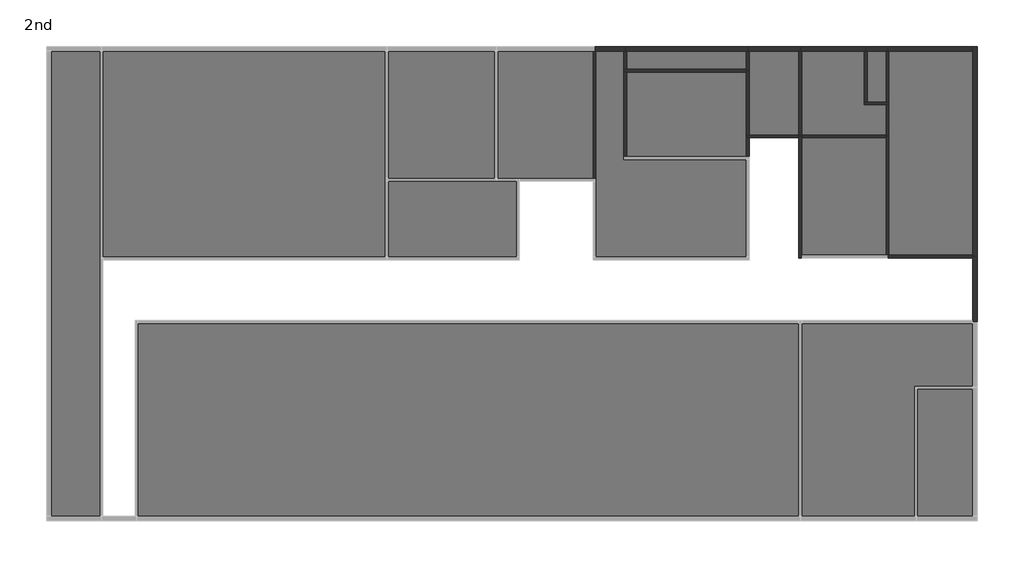
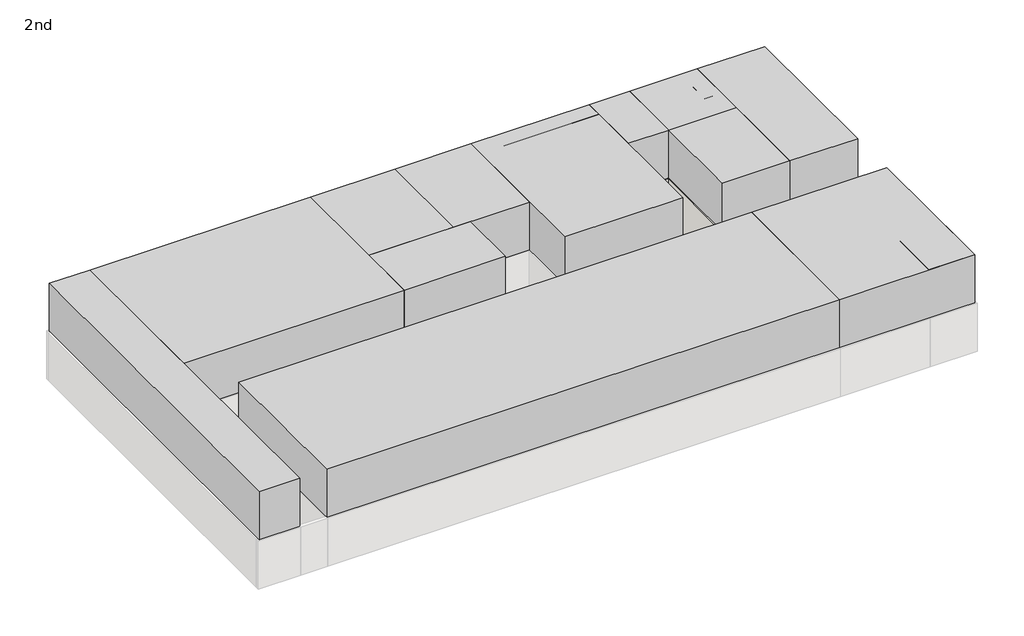
# One storey, part 2 of 2: 42 walls, 17 proxies.
"""IFC4 building model written with IfcOpenShell, lengths in millimetres."""

import ifcopenshell
import ifcopenshell.guid

model = None  # the IFC model being written
_history = None  # IfcOwnerHistory: only IFC2X3 demands one
_inside = {}  # id of a spatial element -> (the spatial element, [elements in it])
_under = {}  # id of a project, library or spatial element -> (it, [spatial elements below it])
_declared = {}  # id of a project -> (the project, [libraries it declares])
_typed = {}  # id of a type object -> (the type object, [elements of that type])
_made_of = {}  # id of a material, layer set ... -> (it, [elements and type objects made of it])


def new_model(schema):
    """Start an empty IFC model of exactly this schema.

    Asked for "IFC4X3", IfcOpenShell would pick the latest addendum, in which some entities
    have other attributes; the version numbers below select the first issue.
    IFC2X3 requires an IfcOwnerHistory on every rooted entity: one is made here for all.
    """
    global model, _history
    if schema == "IFC4X3":
        model = ifcopenshell.file(schema_version=(4, 3, 0, 0))
    else:
        model = ifcopenshell.file(schema=schema)
    _inside.clear()
    _under.clear()
    _declared.clear()
    _typed.clear()
    _made_of.clear()
    _history = None
    if model.schema == "IFC2X3":
        org = make("IfcOrganization", Name="unknown")
        user = make(
            "IfcPersonAndOrganization",
            ThePerson=make("IfcPerson", FamilyName="unknown"),
            TheOrganization=org,
        )
        app = make(
            "IfcApplication",
            ApplicationDeveloper=org,
            Version="unknown",
            ApplicationFullName="unknown",
            ApplicationIdentifier="unknown",
        )
        _history = make(
            "IfcOwnerHistory",
            OwningUser=user,
            OwningApplication=app,
            ChangeAction="ADDED",
            CreationDate=0,
        )
    return model


def make(cls, **values):
    """One entity of the class cls with the attributes given. An attribute that is None is left unset."""
    return model.create_entity(
        cls, **{name: value for name, value in values.items() if value is not None}
    )


def rooted(cls, **values):
    """An entity with a GlobalId (a new one), such as an element, a storey or a relation."""
    return make(cls, GlobalId=ifcopenshell.guid.new(), OwnerHistory=_history, **values)


def si_unit(unit_type, name, prefix=None):
    """IfcSIUnit, for example si_unit("LENGTHUNIT", "METRE", prefix="MILLI")."""
    return make("IfcSIUnit", UnitType=unit_type, Prefix=prefix, Name=name)


def assignment(units):
    """IfcUnitAssignment: the units of a project."""
    return None if units is None else make("IfcUnitAssignment", Units=units)


def point(xyz):
    """IfcCartesianPoint."""
    return None if xyz is None else make("IfcCartesianPoint", Coordinates=xyz)


def direction(xyz):
    """IfcDirection."""
    return None if xyz is None else make("IfcDirection", DirectionRatios=xyz)


def frame(location, z_axis=None, x_axis=None):
    """IfcAxis2Placement3D, a coordinate frame: its origin and axes. An axis left out is left unset."""
    return make(
        "IfcAxis2Placement3D",
        Location=point(location),
        Axis=direction(z_axis),
        RefDirection=direction(x_axis),
    )


def origin():
    """The frame at (0, 0, 0) with its axes left unset."""
    return frame((0.0, 0.0, 0.0))


def origin_with_axes():
    """The frame at (0, 0, 0) with the z axis (0, 0, 1) and the x axis (1, 0, 0) written out."""
    return frame((0.0, 0.0, 0.0), z_axis=(0.0, 0.0, 1.0), x_axis=(1.0, 0.0, 0.0))


def place(relative_to, where):
    """IfcLocalPlacement: puts the frame where relative to a parent placement (None: the world)."""
    return make(
        "IfcLocalPlacement", PlacementRelTo=relative_to, RelativePlacement=where
    )


def context(
    kind, dimensions, precision=None, world=None, true_north=None, identifier=None
):
    """IfcGeometricRepresentationContext, for example the 3D "Model" context."""
    return make(
        "IfcGeometricRepresentationContext",
        ContextIdentifier=identifier,
        ContextType=kind,
        CoordinateSpaceDimension=dimensions,
        Precision=precision,
        WorldCoordinateSystem=world,
        TrueNorth=true_north,
    )


def project(units=None, contexts=None):
    """IfcProject with its units and contexts."""
    return rooted(
        "IfcProject",
        Name="project",
        RepresentationContexts=contexts,
        UnitsInContext=assignment(units),
    )


def spatial(cls, under=None, at=None, **own):
    """A site, building, storey or space (cls), placed at a placement, below another one or the project."""
    s = rooted(cls, ObjectPlacement=at, **own)
    if under is not None:
        _under.setdefault(under.id(), (under, []))[1].append(s)
    return s


def polyline(points):
    """IfcPolyline through the points."""
    return make("IfcPolyline", Points=[point(p) for p in points])


def outline(outer, holes=None, kind="AREA"):
    """IfcArbitraryClosedProfileDef: a profile drawn as a closed curve; with holes, ...WithVoids."""
    if holes is None:
        return make("IfcArbitraryClosedProfileDef", ProfileType=kind, OuterCurve=outer)
    return make(
        "IfcArbitraryProfileDefWithVoids",
        ProfileType=kind,
        OuterCurve=outer,
        InnerCurves=holes,
    )


def extrude(swept, where, along, depth):
    """IfcExtrudedAreaSolid: the profile swept, set in the frame where, extruded along a direction by depth."""
    return make(
        "IfcExtrudedAreaSolid",
        SweptArea=swept,
        Position=where,
        ExtrudedDirection=direction(along),
        Depth=depth,
    )


def faces_of(points, faces, orient=None, outer=None):
    """IfcFace entities. A face is a list of loops; a loop is a list of indices into points, from 0.

    orient and outer hold one flag for each loop. By default every Orientation is true, the
    first loop of a face is its IfcFaceOuterBound and the others are IfcFaceBound.
    """
    made = []
    for i, loops in enumerate(faces):
        bounds = []
        for j, loop in enumerate(loops):
            is_outer = j == 0 if outer is None else outer[i][j]
            bounds.append(
                make(
                    "IfcFaceOuterBound" if is_outer else "IfcFaceBound",
                    Bound=make("IfcPolyLoop", Polygon=[points[k] for k in loop]),
                    Orientation=True if orient is None else orient[i][j],
                )
            )
        made.append(make("IfcFace", Bounds=bounds))
    return made


def faceted_brep(points, faces, orient=None, outer=None, voids=None):
    """IfcFacetedBrep: a solid bounded by flat faces; with voids (closed shells), ...WithVoids."""
    shared = [point(p) for p in points]
    hull = make("IfcClosedShell", CfsFaces=faces_of(shared, faces, orient, outer))
    if voids is None:
        return make("IfcFacetedBrep", Outer=hull)
    return make(
        "IfcFacetedBrepWithVoids",
        Outer=hull,
        Voids=[
            make(cls, CfsFaces=faces_of(shared, fs, o, b)) for cls, fs, o, b in voids
        ],
    )


def shape(context_of_items, identifier, shape_type, items):
    """IfcShapeRepresentation: the items that make up one representation, for example the "Body"."""
    return make(
        "IfcShapeRepresentation",
        ContextOfItems=context_of_items,
        RepresentationIdentifier=identifier,
        RepresentationType=shape_type,
        Items=items,
    )


def source(mapping_origin, context_of_items, identifier, shape_type, items):
    """IfcRepresentationMap: a shape defined once, which mapped items show again and again."""
    return make(
        "IfcRepresentationMap",
        MappingOrigin=mapping_origin,
        MappedRepresentation=shape(context_of_items, identifier, shape_type, items),
    )


def transform(
    local_origin,
    x_axis=None,
    y_axis=None,
    z_axis=None,
    scale=None,
    scale2=None,
    scale3=None,
    uniform=True,
):
    """IfcCartesianTransformationOperator3D, or its non-uniform kind. x_axis, y_axis, z_axis: its Axis1, 2, 3."""
    if uniform:
        return make(
            "IfcCartesianTransformationOperator3D",
            Axis1=direction(x_axis),
            Axis2=direction(y_axis),
            LocalOrigin=point(local_origin),
            Scale=scale,
            Axis3=direction(z_axis),
        )
    return make(
        "IfcCartesianTransformationOperator3DnonUniform",
        Axis1=direction(x_axis),
        Axis2=direction(y_axis),
        LocalOrigin=point(local_origin),
        Scale=scale,
        Axis3=direction(z_axis),
        Scale2=scale2,
        Scale3=scale3,
    )


def mapped(mapping_source, mapping_target):
    """IfcMappedItem: shows the shape of a source again, moved by a transform."""
    return make(
        "IfcMappedItem", MappingSource=mapping_source, MappingTarget=mapping_target
    )


def made_of(thing, what):
    """Note that an element or type object is made of a material, layer set ...; save() writes the relation."""
    if what is not None:
        _made_of.setdefault(what.id(), (what, []))[1].append(thing)
    return thing


def element(
    cls,
    number,
    at=None,
    inside=None,
    cuts=None,
    type_object=None,
    material=None,
    context=None,
    identifier="Body",
    shape_type=None,
    held_by="IfcProductDefinitionShape",
    body=None,
    shapes=None,
    **own,
):
    """One element of the class cls, such as IfcWall. Its Tag is "e" and its number.

    at: its placement. inside: the storey or other place that contains it. cuts: it is an
    opening in that element (IfcRelVoidsElement). A single representation is given by context,
    identifier, shape_type and body (its items); several are given by shapes. held_by: the class
    of the entity that holds the representations. save() writes the other relations.
    """
    e = rooted(cls, Tag="e%d" % number, ObjectPlacement=at, **own)
    if body is not None:
        shapes = [shape(context, identifier, shape_type, body)]
    if shapes is not None:
        e.Representation = make(held_by, Representations=shapes)
    if inside is not None:
        _inside.setdefault(inside.id(), (inside, []))[1].append(e)
    if cuts is not None:
        rooted(
            "IfcRelVoidsElement", RelatingBuildingElement=cuts, RelatedOpeningElement=e
        )
    if type_object is not None:
        _typed.setdefault(type_object.id(), (type_object, []))[1].append(e)
    return made_of(e, material)


def aggregate(whole, parts):
    """IfcRelAggregates: a whole, such as a stair, and the parts it consists of."""
    return rooted("IfcRelAggregates", RelatingObject=whole, RelatedObjects=parts)


def save(model, path):
    """Write the relations noted so far, then the file.

    IfcRelAggregates (storeys below a building ...), IfcRelContainedInSpatialStructure (elements
    in a storey), IfcRelDefinesByType, IfcRelAssociatesMaterial and IfcRelDeclares: one each for
    every whole, place, type object, material and project.
    """
    for whole, parts in _under.values():
        aggregate(whole, parts)
    for where, things in _inside.values():
        rooted(
            "IfcRelContainedInSpatialStructure",
            RelatedElements=things,
            RelatingStructure=where,
        )
    for kind, things in _typed.values():
        rooted("IfcRelDefinesByType", RelatedObjects=things, RelatingType=kind)
    for what, things in _made_of.values():
        rooted("IfcRelAssociatesMaterial", RelatedObjects=things, RelatingMaterial=what)
    for by, libraries in _declared.values():
        rooted("IfcRelDeclares", RelatingContext=by, RelatedDefinitions=libraries)
    model.write(path)


def space_planning_box_space_planning_box_5634f436(model_context):
    return source(origin(), model_context, "Body", "SweptSolid", [
        extrude(outline(polyline([(1350.0, 3000.0), (1350.0, -3000.0), (-1350.0, -3000.0), (-1350.0, 3000.0), (1350.0, 3000.0)])), origin_with_axes(), (0.0, 0.0, 1.0), 6000.0),
    ])


def space_planning_box_space_planning_box_71e2440f(model_context):
    return source(origin(), model_context, "Body", "SweptSolid", [
        extrude(outline(polyline([(500.0, 1250.0), (500.0, -1250.0), (-500.0, -1250.0), (-500.0, 1250.0), (500.0, 1250.0)])), origin_with_axes(), (0.0, 0.0, 1.0), 6000.0),
    ])


def space_planning_box_space_planning_box_ce7d2093(model_context):
    return source(origin(), model_context, "Body", "SweptSolid", [
        extrude(outline(polyline([(4500.0, 15175.0), (4500.0, -15175.0), (-4500.0, -15175.0), (-4500.0, 15175.0), (4500.0, 15175.0)])), origin_with_axes(), (0.0, 0.0, 1.0), 6000.0),
    ])


def space_planning_box_space_planning_box_c2e9f8fb(model_context):
    return source(origin(), model_context, "Body", "SweptSolid", [
        extrude(outline(polyline([(4800.0, 6525.0), (4800.0, -6525.0), (-4800.0, -6525.0), (-4800.0, 6525.0), (4800.0, 6525.0)])), origin_with_axes(), (0.0, 0.0, 1.0), 6000.0),
    ])


def space_planning_box_space_planning_box_44ef6168(model_context):
    return source(origin(), model_context, "Body", "SweptSolid", [
        extrude(outline(polyline([(2500.0, 3000.0), (2500.0, -3000.0), (-2500.0, -3000.0), (-2500.0, 3000.0), (2500.0, 3000.0)])), origin_with_axes(), (0.0, 0.0, 1.0), 6000.0),
    ])


def space_planning_box_space_planning_box_4d084078(model_context):
    return source(origin(), model_context, "Body", "SweptSolid", [
        extrude(outline(polyline([(4000.0, 4500.0), (4000.0, -4500.0), (-4000.0, -4500.0), (-4000.0, 4500.0), (4000.0, 4500.0)])), origin_with_axes(), (0.0, 0.0, 1.0), 6000.0),
    ])


def space_planning_box_space_planning_box_072414e0(model_context):
    return source(origin(), model_context, "Body", "SweptSolid", [
        extrude(outline(polyline([(3500.0, 4800.0), (3500.0, -4800.0), (-3500.0, -4800.0), (-3500.0, 4800.0), (3500.0, 4800.0)])), origin_with_axes(), (0.0, 0.0, 1.0), 6000.0),
    ])


def space_planning_box_space_planning_box_34e84c64(model_context):
    return source(origin(), model_context, "Body", "SweptSolid", [
        extrude(outline(polyline([(2750.0, 2000.0), (2750.0, -2000.0), (-2750.0, -2000.0), (-2750.0, 2000.0), (2750.0, 2000.0)])), origin_with_axes(), (0.0, 0.0, 1.0), 6000.0),
    ])


def space_planning_box_space_planning_box_7bff30ad(model_context):
    return source(origin(), model_context, "Body", "SweptSolid", [
        extrude(outline(polyline([(2000.0, 2000.0), (2000.0, -2000.0), (-2000.0, -2000.0), (-2000.0, 2000.0), (2000.0, 2000.0)])), origin_with_axes(), (0.0, 0.0, 1.0), 6000.0),
    ])


def space_planning_box_space_planning_box_03407eb8(model_context):
    return source(origin(), model_context, "Body", "SweptSolid", [
        extrude(outline(polyline([(1200.0, 10750.0), (1200.0, -10750.0), (-1200.0, -10750.0), (-1200.0, 10750.0), (1200.0, 10750.0)])), origin_with_axes(), (0.0, 0.0, 1.0), 6000.0),
    ])


def space_planning_box_space_planning_box_3a820573(model_context):
    return source(origin(), model_context, "Body", "SweptSolid", [
        extrude(outline(polyline([(2000.0, 4750.0), (2000.0, -4750.0), (-2000.0, -4750.0), (-2000.0, 4750.0), (2000.0, 4750.0)])), origin_with_axes(), (0.0, 0.0, 1.0), 6000.0),
    ])


def space_planning_box_space_planning_box_8af91fed(model_context):
    return source(origin(), model_context, "Body", "SweptSolid", [
        extrude(outline(polyline([(2250.0, 3000.0), (2250.0, -3000.0), (-2250.0, -3000.0), (-2250.0, 3000.0), (2250.0, 3000.0)])), origin_with_axes(), (0.0, 0.0, 1.0), 6000.0),
    ])


def space_planning_box_space_planning_box_837d2e24(model_context):
    return source(origin(), model_context, "Body", "SweptSolid", [
        extrude(outline(polyline([(1800.0, 3000.0), (1800.0, -3000.0), (-1800.0, -3000.0), (-1800.0, 3000.0), (1800.0, 3000.0)])), origin_with_axes(), (0.0, 0.0, 1.0), 6000.0),
    ])


def space_planning_box_space_planning_box_47b98be1(model_context):
    return source(origin(), model_context, "Body", "SweptSolid", [
        extrude(outline(polyline([(1200.0, 2000.0), (1200.0, -2000.0), (-1200.0, -2000.0), (-1200.0, 2000.0), (1200.0, 2000.0)])), origin_with_axes(), (0.0, 0.0, 1.0), 6000.0),
    ])


def space_planning_box_space_planning_box_a556ef48(model_context):
    return source(origin(), model_context, "Body", "SweptSolid", [
        extrude(outline(polyline([(500.0, 2800.0), (500.0, -2800.0), (-500.0, -2800.0), (-500.0, 2800.0), (500.0, 2800.0)])), origin_with_axes(), (0.0, 0.0, 1.0), 6000.0),
    ])


def space_planning_box_space_planning_box_c1734578(model_context):
    return source(origin(), model_context, "Body", "SweptSolid", [
        extrude(outline(polyline([(2800.0, 2500.0), (2800.0, -2500.0), (-2800.0, -2500.0), (-2800.0, 2500.0), (2800.0, 2500.0)])), origin_with_axes(), (0.0, 0.0, 1.0), 6000.0),
    ])


model = new_model("IFC4")

# Units and contexts
model_context = context("Model", 3, world=origin())
ifc_project = project(units=[si_unit("LENGTHUNIT", "METRE", prefix="MILLI")], contexts=[model_context])

# Site, building, storey
site = spatial("IfcSite", under=ifc_project)
building = spatial("IfcBuilding", under=site)
storey = spatial("IfcBuildingStorey", under=building, Name="2nd", Elevation=14000.0)

# Proxies
placement = place(None, origin())
space_planning_box_space_planning_box_shape = space_planning_box_space_planning_box_5634f436(model_context)
element("IfcBuildingElementProxy", 1, Name="Space Planning Box : Space Planning Box", ObjectType="Space Planning Box : Space Planning Box", at=placement, inside=storey, context=model_context, shape_type="MappedRepresentation", body=[
    mapped(space_planning_box_space_planning_box_shape, transform((48750.0, 154250.0, 14000.0), x_axis=(1.0, 0.0, 0.0), y_axis=(0.0, 1.0, 0.0), z_axis=(0.0, 0.0, 1.0))),
])
space_planning_box_space_planning_box_2_shape = space_planning_box_space_planning_box_71e2440f(model_context)
element("IfcBuildingElementProxy", 2, Name="Space Planning Box : Space Planning Box", ObjectType="Space Planning Box : Space Planning Box", at=placement, inside=storey, context=model_context, shape_type="MappedRepresentation", body=[
    mapped(space_planning_box_space_planning_box_2_shape, transform((45600.0, 171500.0, 14000.0), x_axis=(1.0, 0.0, 0.0), y_axis=(0.0, 1.0, 0.0), z_axis=(0.0, 0.0, 1.0))),
])
space_planning_box_space_planning_box_3_shape = space_planning_box_space_planning_box_ce7d2093(model_context)
element("IfcBuildingElementProxy", 3, Name="Space Planning Box : Space Planning Box", ObjectType="Space Planning Box : Space Planning Box", at=placement, inside=storey, context=model_context, shape_type="MappedRepresentation", body=[
    mapped(space_planning_box_space_planning_box_3_shape, transform((26925.0, 155750.0, 14000.0), x_axis=(0.0, -1.0, 0.0), y_axis=(1.0, 0.0, 0.0), z_axis=(0.0, 0.0, 1.0))),
])
space_planning_box_space_planning_box_4_shape = space_planning_box_space_planning_box_c2e9f8fb(model_context)
element("IfcBuildingElementProxy", 4, Name="Space Planning Box : Space Planning Box", ObjectType="Space Planning Box : Space Planning Box", at=placement, inside=storey, context=model_context, shape_type="MappedRepresentation", body=[
    mapped(space_planning_box_space_planning_box_4_shape, transform((16675.0, 167950.0, 14000.0), x_axis=(0.0, -1.0, 0.0), y_axis=(1.0, 0.0, 0.0), z_axis=(0.0, 0.0, 1.0))),
])
space_planning_box_space_planning_box_5_shape = space_planning_box_space_planning_box_44ef6168(model_context)
element("IfcBuildingElementProxy", 5, Name="Space Planning Box : Space Planning Box", ObjectType="Space Planning Box : Space Planning Box", at=placement, inside=storey, context=model_context, shape_type="MappedRepresentation", body=[
    mapped(space_planning_box_space_planning_box_5_shape, transform((25700.0, 169750.0, 14000.0), x_axis=(1.0, 0.0, 0.0), y_axis=(0.0, 1.0, 0.0), z_axis=(0.0, 0.0, 1.0))),
])
space_planning_box_space_planning_box_6_shape = space_planning_box_space_planning_box_4d084078(model_context)
element("IfcBuildingElementProxy", 6, Name="Space Planning Box : Space Planning Box", ObjectType="Space Planning Box : Space Planning Box", at=placement, inside=storey, context=model_context, shape_type="MappedRepresentation", body=[
    mapped(space_planning_box_space_planning_box_6_shape, transform((46100.0, 155750.0, 14000.0), x_axis=(1.0, 0.0, 0.0), y_axis=(0.0, 1.0, 0.0), z_axis=(0.0, 0.0, 1.0))),
])
space_planning_box_space_planning_box_7_shape = space_planning_box_space_planning_box_072414e0(model_context)
element("IfcBuildingElementProxy", 7, Name="Space Planning Box : Space Planning Box", ObjectType="Space Planning Box : Space Planning Box", at=placement, inside=storey, context=model_context, shape_type="MappedRepresentation", body=[
    mapped(space_planning_box_space_planning_box_7_shape, transform((36200.0, 167950.0, 14000.0), x_axis=(1.0, 0.0, 0.0), y_axis=(0.0, 1.0, 0.0), z_axis=(0.0, 0.0, 1.0))),
])
space_planning_box_space_planning_box_8_shape = space_planning_box_space_planning_box_34e84c64(model_context)
element("IfcBuildingElementProxy", 8, Name="Space Planning Box : Space Planning Box", ObjectType="Space Planning Box : Space Planning Box", at=placement, inside=storey, context=model_context, shape_type="MappedRepresentation", body=[
    mapped(space_planning_box_space_planning_box_8_shape, transform((44100.0, 166000.0, 14000.0), x_axis=(0.0, -1.0, 0.0), y_axis=(1.0, 0.0, 0.0), z_axis=(0.0, 0.0, 1.0))),
])
space_planning_box_space_planning_box_9_shape = space_planning_box_space_planning_box_7bff30ad(model_context)
element("IfcBuildingElementProxy", 9, Name="Space Planning Box : Space Planning Box", ObjectType="Space Planning Box : Space Planning Box", at=placement, inside=storey, context=model_context, shape_type="MappedRepresentation", body=[
    mapped(space_planning_box_space_planning_box_9_shape, transform((44100.0, 170750.0, 14000.0), x_axis=(1.0, 0.0, 0.0), y_axis=(0.0, 1.0, 0.0), z_axis=(0.0, 0.0, 1.0))),
])
space_planning_box_space_planning_box_10_shape = space_planning_box_space_planning_box_03407eb8(model_context)
element("IfcBuildingElementProxy", 10, Name="Space Planning Box : Space Planning Box", ObjectType="Space Planning Box : Space Planning Box", at=placement, inside=storey, context=model_context, shape_type="MappedRepresentation", body=[
    mapped(space_planning_box_space_planning_box_10_shape, transform((8950.0, 162000.0, 14000.0), x_axis=(1.0, 0.0, 0.0), y_axis=(0.0, 1.0, 0.0), z_axis=(0.0, 0.0, 1.0))),
])
space_planning_box_space_planning_box_11_shape = space_planning_box_space_planning_box_3a820573(model_context)
element("IfcBuildingElementProxy", 11, Name="Space Planning Box : Space Planning Box", ObjectType="Space Planning Box : Space Planning Box", at=placement, inside=storey, context=model_context, shape_type="MappedRepresentation", body=[
    mapped(space_planning_box_space_planning_box_11_shape, transform((48100.0, 168000.0, 14000.0), x_axis=(1.0, 0.0, 0.0), y_axis=(0.0, 1.0, 0.0), z_axis=(0.0, 0.0, 1.0))),
])
space_planning_box_space_planning_box_12_shape = space_planning_box_space_planning_box_8af91fed(model_context)
element("IfcBuildingElementProxy", 12, Name="Space Planning Box : Space Planning Box", ObjectType="Space Planning Box : Space Planning Box", at=placement, inside=storey, context=model_context, shape_type="MappedRepresentation", body=[
    mapped(space_planning_box_space_planning_box_12_shape, transform((30450.0, 169750.0, 14000.0), x_axis=(1.0, 0.0, 0.0), y_axis=(0.0, 1.0, 0.0), z_axis=(0.0, 0.0, 1.0))),
])
space_planning_box_space_planning_box_13_shape = space_planning_box_space_planning_box_837d2e24(model_context)
element("IfcBuildingElementProxy", 13, Name="Space Planning Box : Space Planning Box", ObjectType="Space Planning Box : Space Planning Box", at=placement, inside=storey, context=model_context, shape_type="MappedRepresentation", body=[
    mapped(space_planning_box_space_planning_box_13_shape, transform((26200.0, 164950.0, 14000.0), x_axis=(0.0, -1.0, 0.0), y_axis=(1.0, 0.0, 0.0), z_axis=(0.0, 0.0, 1.0))),
])
space_planning_box_space_planning_box_14_shape = space_planning_box_space_planning_box_47b98be1(model_context)
element("IfcBuildingElementProxy", 14, Name="Space Planning Box : Space Planning Box", ObjectType="Space Planning Box : Space Planning Box", at=placement, inside=storey, context=model_context, shape_type="MappedRepresentation", body=[
    mapped(space_planning_box_space_planning_box_14_shape, transform((40900.0, 170750.0, 14000.0), x_axis=(1.0, 0.0, 0.0), y_axis=(0.0, 1.0, 0.0), z_axis=(0.0, 0.0, 1.0))),
])
element("IfcBuildingElementProxy", 15, Name="Space Planning Box : Space Planning Box", ObjectType="Space Planning Box : Space Planning Box", at=placement, inside=storey, context=model_context, shape_type="MappedRepresentation", body=[
    mapped(space_planning_box_space_planning_box_14_shape, transform((40900.0, 170750.0, 14000.0), x_axis=(1.0, 0.0, 0.0), y_axis=(0.0, 1.0, 0.0), z_axis=(0.0, 0.0, 1.0))),
])
space_planning_box_space_planning_box_15_shape = space_planning_box_space_planning_box_a556ef48(model_context)
element("IfcBuildingElementProxy", 16, Name="Space Planning Box : Space Planning Box", ObjectType="Space Planning Box : Space Planning Box", at=placement, inside=storey, context=model_context, shape_type="MappedRepresentation", body=[
    mapped(space_planning_box_space_planning_box_15_shape, transform((36900.0, 172250.0, 14000.0), x_axis=(0.0, 1.0, 0.0), y_axis=(-1.0, 0.0, 0.0), z_axis=(0.0, 0.0, 1.0))),
])
space_planning_box_space_planning_box_16_shape = space_planning_box_space_planning_box_c1734578(model_context)
element("IfcBuildingElementProxy", 17, Name="Space Planning Box : Space Planning Box", ObjectType="Space Planning Box : Space Planning Box", at=placement, inside=storey, context=model_context, shape_type="MappedRepresentation", body=[
    mapped(space_planning_box_space_planning_box_16_shape, transform((36900.0, 170250.0, 14000.0), x_axis=(1.0, 0.0, 0.0), y_axis=(0.0, 1.0, 0.0), z_axis=(0.0, 0.0, 1.0))),
])

# Walls
element("IfcWall", 18, ObjectType="Wall-Ext_215Bwk", at=placement, inside=storey, context=model_context, shape_type="Brep", body=[
    faceted_brep([(49992.5, 172857.5, 14000.0), (46100.0, 172857.5, 14000.0), (46100.0, 172857.5, 17000.0), (49992.5, 172857.5, 17000.0), (49992.5, 172642.5, 14000.0), (49992.5, 172642.5, 17000.0), (46162.5, 172642.5, 17000.0), (46100.0, 172642.5, 17000.0), (46100.0, 172642.5, 14000.0), (46162.5, 172642.5, 14000.0)], [[[0, 1, 2, 3]], [[4, 5, 6, 7, 8, 9]], [[1, 0, 4, 9, 8]], [[2, 1, 8, 7]], [[3, 2, 7, 6, 5]], [[0, 3, 5, 4]]]),
])
element("IfcWall", 19, ObjectType="Wall-Ext_215Bwk", at=placement, inside=storey, context=model_context, shape_type="Brep", body=[
    faceted_brep([(50207.5, 163250.0, 14000.0), (50207.5, 172857.5, 14000.0), (50207.5, 172857.5, 17000.0), (50207.5, 163250.0, 17000.0), (49992.5, 163250.0, 14000.0), (49992.5, 163250.0, 17000.0), (49992.5, 163312.5, 17000.0), (49992.5, 172642.5, 17000.0), (49992.5, 172857.5, 17000.0), (49992.5, 172857.5, 14000.0), (49992.5, 172642.5, 14000.0), (49992.5, 163312.5, 14000.0)], [[[0, 1, 2, 3]], [[4, 5, 6, 7, 8, 9, 10, 11]], [[1, 0, 4, 11, 10, 9]], [[3, 2, 8, 7, 6, 5]], [[0, 3, 5, 4]], [[2, 1, 9, 8]]]),
])
element("IfcWall", 20, ObjectType="Wall-Ext_215Bwk", at=placement, inside=storey, context=model_context, shape_type="Brep", body=[
    faceted_brep([(42100.0, 172857.5, 14000.0), (39700.0, 172857.5, 14000.0), (39700.0, 172857.5, 17000.0), (42100.0, 172857.5, 17000.0), (42100.0, 172642.5, 14000.0), (42100.0, 172642.5, 17000.0), (42037.5, 172642.5, 17000.0), (39762.5, 172642.5, 17000.0), (39700.0, 172642.5, 17000.0), (39700.0, 172642.5, 14000.0), (39762.5, 172642.5, 14000.0), (42037.5, 172642.5, 14000.0)], [[[0, 1, 2, 3]], [[4, 5, 6, 7, 8, 9, 10, 11]], [[1, 0, 4, 11, 10, 9]], [[2, 1, 9, 8]], [[3, 2, 8, 7, 6, 5]], [[0, 3, 5, 4]]]),
])
element("IfcWall", 21, ObjectType="Wall-Ext_215Bwk", at=placement, inside=storey, context=model_context, shape_type="Brep", body=[
    faceted_brep([(39700.0, 172857.5, 14000.0), (34100.0, 172857.5, 14000.0), (34100.0, 172857.5, 17000.0), (39700.0, 172857.5, 17000.0), (39700.0, 172642.5, 14000.0), (39700.0, 172642.5, 17000.0), (39637.5, 172642.5, 17000.0), (34162.5, 172642.5, 17000.0), (34100.0, 172642.5, 17000.0), (34100.0, 172642.5, 14000.0), (34162.5, 172642.5, 14000.0), (39637.5, 172642.5, 14000.0)], [[[0, 1, 2, 3]], [[4, 5, 6, 7, 8, 9, 10, 11]], [[1, 0, 4, 11, 10, 9]], [[2, 1, 9, 8]], [[3, 2, 8, 7, 6, 5]], [[0, 3, 5, 4]]]),
])
element("IfcWall", 22, ObjectType="Wall-Ext_215Bwk", at=placement, inside=storey, context=model_context, shape_type="Brep", body=[
    faceted_brep([(34100.0, 172857.5, 14000.0), (32700.0, 172857.5, 14000.0), (32700.0, 172857.5, 17000.0), (34100.0, 172857.5, 17000.0), (34100.0, 172642.5, 14000.0), (34100.0, 172642.5, 17000.0), (34037.5, 172642.5, 17000.0), (32762.5, 172642.5, 17000.0), (32700.0, 172642.5, 17000.0), (32700.0, 172642.5, 14000.0), (32762.5, 172642.5, 14000.0), (34037.5, 172642.5, 14000.0)], [[[0, 1, 2, 3]], [[4, 5, 6, 7, 8, 9, 10, 11]], [[1, 0, 4, 11, 10, 9]], [[2, 1, 9, 8]], [[3, 2, 8, 7, 6, 5]], [[0, 3, 5, 4]]]),
])
element("IfcWall", 23, ObjectType="Wall-Ext_215Bwk", at=placement, inside=storey, context=model_context, shape_type="Brep", body=[
    faceted_brep([(45100.0, 172857.5, 14000.0), (42100.0, 172857.5, 14000.0), (42100.0, 172857.5, 17000.0), (45100.0, 172857.5, 17000.0), (45100.0, 172642.5, 14000.0), (45100.0, 172642.5, 17000.0), (45037.5, 172642.5, 17000.0), (42162.5, 172642.5, 17000.0), (42100.0, 172642.5, 17000.0), (42100.0, 172642.5, 14000.0), (42162.5, 172642.5, 14000.0), (45037.5, 172642.5, 14000.0)], [[[0, 1, 2, 3]], [[4, 5, 6, 7, 8, 9, 10, 11]], [[1, 0, 4, 11, 10, 9]], [[2, 1, 9, 8]], [[3, 2, 8, 7, 6, 5]], [[0, 3, 5, 4]]]),
])
element("IfcWall", 24, ObjectType="Wall-Ext_215Bwk", at=placement, inside=storey, context=model_context, shape_type="Brep", body=[
    faceted_brep([(46100.0, 172857.5, 14000.0), (45100.0, 172857.5, 14000.0), (45100.0, 172857.5, 17000.0), (46100.0, 172857.5, 17000.0), (46100.0, 172642.5, 14000.0), (46100.0, 172642.5, 17000.0), (46037.5, 172642.5, 17000.0), (45162.5, 172642.5, 17000.0), (45100.0, 172642.5, 17000.0), (45100.0, 172642.5, 14000.0), (45162.5, 172642.5, 14000.0), (46037.5, 172642.5, 14000.0)], [[[0, 1, 2, 3]], [[4, 5, 6, 7, 8, 9, 10, 11]], [[1, 0, 4, 11, 10, 9]], [[2, 1, 9, 8]], [[3, 2, 8, 7, 6, 5]], [[0, 3, 5, 4]]]),
])
element("IfcWall", 25, ObjectType="Wall-Ext_215Bwk", at=placement, inside=storey, context=model_context, shape_type="Brep", body=[
    faceted_brep([(50207.5, 160250.0, 14000.0), (50207.5, 163250.0, 14000.0), (50207.5, 163250.0, 17000.0), (50207.5, 160250.0, 17000.0), (49992.5, 160250.0, 14000.0), (49992.5, 160250.0, 17000.0), (49992.5, 160312.5, 17000.0), (49992.5, 163187.5, 17000.0), (49992.5, 163250.0, 17000.0), (49992.5, 163250.0, 14000.0), (49992.5, 163187.5, 14000.0), (49992.5, 160312.5, 14000.0)], [[[0, 1, 2, 3]], [[4, 5, 6, 7, 8, 9, 10, 11]], [[1, 0, 4, 11, 10, 9]], [[2, 1, 9, 8]], [[3, 2, 8, 7, 6, 5]], [[0, 3, 5, 4]]]),
])
element("IfcWall", 26, ObjectType="Wall-Int_12P-100Blk-12P", at=placement, inside=storey, context=model_context, shape_type="Brep", body=[
    faceted_brep([(46037.5, 168812.5, 14000.0), (42162.5, 168812.5, 14000.0), (42162.5, 168812.5, 17000.0), (46037.5, 168812.5, 17000.0), (46037.5, 168687.5, 14000.0), (46037.5, 168687.5, 17000.0), (42162.5, 168687.5, 17000.0), (42162.5, 168687.5, 14000.0), (46037.5, 168750.0, 14000.0), (42162.5, 168750.0, 14000.0), (42162.5, 168750.0, 17000.0), (46037.5, 168750.0, 17000.0)], [[[0, 1, 2, 3]], [[4, 5, 6, 7]], [[1, 0, 8, 4, 7, 9]], [[3, 2, 10, 6, 5, 11]], [[0, 3, 11, 5, 4, 8]], [[2, 1, 9, 7, 6, 10]]]),
])
element("IfcWall", 27, ObjectType="Wall-Int_12P-100Blk-12P", at=placement, inside=storey, context=model_context, shape_type="Brep", body=[
    faceted_brep([(42037.5, 168750.0, 14000.0), (42037.5, 168687.5, 14000.0), (42037.5, 163187.5, 14000.0), (42037.5, 163187.5, 17000.0), (42037.5, 168687.5, 17000.0), (42037.5, 168750.0, 17000.0), (42162.5, 168750.0, 14000.0), (42162.5, 168750.0, 17000.0), (42162.5, 168687.5, 17000.0), (42162.5, 163312.5, 17000.0), (42162.5, 163187.5, 17000.0), (42162.5, 163187.5, 14000.0), (42162.5, 163312.5, 14000.0), (42162.5, 168687.5, 14000.0)], [[[0, 1, 2, 3, 4, 5]], [[6, 7, 8, 9, 10, 11, 12, 13]], [[2, 1, 0, 6, 13, 12, 11]], [[5, 4, 3, 10, 9, 8, 7]], [[0, 5, 7, 6]], [[3, 2, 11, 10]]]),
])
element("IfcWall", 28, ObjectType="Wall-Int_12P-100Blk-12P", at=placement, inside=storey, context=model_context, shape_type="Brep", body=[
    faceted_brep([(46162.5, 163312.5, 14000.0), (46162.5, 168750.0, 14000.0), (46162.5, 168750.0, 17000.0), (46162.5, 163312.5, 17000.0), (46037.5, 163312.5, 14000.0), (46037.5, 163312.5, 17000.0), (46037.5, 168687.5, 17000.0), (46037.5, 168750.0, 17000.0), (46037.5, 168750.0, 14000.0), (46037.5, 168687.5, 14000.0), (46100.0, 163312.5, 14000.0), (46100.0, 163312.5, 17000.0)], [[[0, 1, 2, 3]], [[4, 5, 6, 7, 8, 9]], [[1, 0, 10, 4, 9, 8]], [[2, 1, 8, 7]], [[3, 2, 7, 6, 5, 11]], [[0, 3, 11, 5, 4, 10]]]),
])
element("IfcWall", 29, ObjectType="Wall-Int_12P-100Blk-12P", at=placement, inside=storey, context=model_context, shape_type="Brep", body=[
    faceted_brep([(46037.5, 168750.0, 14000.0), (46037.5, 168687.5, 14000.0), (46037.5, 163312.5, 14000.0), (46037.5, 163312.5, 17000.0), (46037.5, 168687.5, 17000.0), (46037.5, 168750.0, 17000.0), (46162.5, 168750.0, 14000.0), (46162.5, 168750.0, 17000.0), (46162.5, 163312.5, 17000.0), (46162.5, 163312.5, 14000.0), (46100.0, 163312.5, 14000.0), (46100.0, 163312.5, 17000.0)], [[[0, 1, 2, 3, 4, 5]], [[6, 7, 8, 9]], [[2, 1, 0, 6, 9, 10]], [[5, 4, 3, 11, 8, 7]], [[0, 5, 7, 6]], [[3, 2, 10, 9, 8, 11]]]),
])
element("IfcWall", 30, ObjectType="Wall-Int_12P-100Blk-12P", at=placement, inside=storey, context=model_context, shape_type="Brep", body=[
    faceted_brep([(46100.0, 163187.5, 14000.0), (49992.5, 163187.5, 14000.0), (49992.5, 163187.5, 17000.0), (46100.0, 163187.5, 17000.0), (46100.0, 163312.5, 14000.0), (46100.0, 163312.5, 17000.0), (46162.5, 163312.5, 17000.0), (49992.5, 163312.5, 17000.0), (49992.5, 163312.5, 14000.0), (46162.5, 163312.5, 14000.0), (49992.5, 163250.0, 14000.0), (49992.5, 163250.0, 17000.0)], [[[0, 1, 2, 3]], [[4, 5, 6, 7, 8, 9]], [[1, 0, 4, 9, 8, 10]], [[3, 2, 11, 7, 6, 5]], [[0, 3, 5, 4]], [[2, 1, 10, 8, 7, 11]]]),
])
element("IfcWall", 31, ObjectType="Wall-Int_12P-100Blk-12P", at=placement, inside=storey, context=model_context, shape_type="Brep", body=[
    faceted_brep([(46037.5, 172642.5, 14000.0), (46037.5, 170312.5, 14000.0), (46037.5, 170312.5, 17000.0), (46037.5, 172642.5, 17000.0), (46162.5, 172642.5, 14000.0), (46162.5, 172642.5, 17000.0), (46162.5, 170312.5, 17000.0), (46162.5, 170312.5, 14000.0), (46100.0, 172642.5, 14000.0), (46100.0, 172642.5, 17000.0)], [[[0, 1, 2, 3]], [[4, 5, 6, 7]], [[1, 0, 8, 4, 7]], [[3, 2, 6, 5, 9]], [[2, 1, 7, 6]], [[0, 3, 9, 5, 4, 8]]]),
])
element("IfcWall", 32, ObjectType="Wall-Int_12P-100Blk-12P", at=placement, inside=storey, context=model_context, shape_type="Brep", body=[
    faceted_brep([(46037.5, 170187.5, 14000.0), (46037.5, 168812.5, 14000.0), (46037.5, 168750.0, 14000.0), (46037.5, 168750.0, 17000.0), (46037.5, 168812.5, 17000.0), (46037.5, 170187.5, 17000.0), (46162.5, 170187.5, 14000.0), (46162.5, 170187.5, 17000.0), (46162.5, 168750.0, 17000.0), (46162.5, 168750.0, 14000.0)], [[[0, 1, 2, 3, 4, 5]], [[6, 7, 8, 9]], [[2, 1, 0, 6, 9]], [[3, 2, 9, 8]], [[5, 4, 3, 8, 7]], [[0, 5, 7, 6]]]),
])
element("IfcWall", 33, ObjectType="Wall-Int_12P-100Blk-12P", at=placement, inside=storey, context=model_context, shape_type="Brep", body=[
    faceted_brep([(32762.5, 166812.5, 14000.0), (32762.5, 172642.5, 14000.0), (32762.5, 172642.5, 17000.0), (32762.5, 166812.5, 17000.0), (32637.5, 166812.5, 14000.0), (32637.5, 166812.5, 17000.0), (32637.5, 172642.5, 17000.0), (32637.5, 172642.5, 14000.0), (32700.0, 172642.5, 14000.0), (32700.0, 172642.5, 17000.0)], [[[0, 1, 2, 3]], [[4, 5, 6, 7]], [[1, 0, 4, 7, 8]], [[3, 2, 9, 6, 5]], [[0, 3, 5, 4]], [[2, 1, 8, 7, 6, 9]]]),
])
element("IfcWall", 34, ObjectType="Wall-Int_12P-100Blk-12P", at=placement, inside=storey, context=model_context, shape_type="Brep", body=[
    faceted_brep([(39637.5, 172642.5, 14000.0), (39637.5, 171812.5, 14000.0), (39637.5, 171750.0, 14000.0), (39637.5, 171750.0, 17000.0), (39637.5, 171812.5, 17000.0), (39637.5, 172642.5, 17000.0), (39762.5, 172642.5, 14000.0), (39762.5, 172642.5, 17000.0), (39762.5, 171750.0, 17000.0), (39762.5, 171750.0, 14000.0), (39700.0, 172642.5, 14000.0), (39700.0, 172642.5, 17000.0)], [[[0, 1, 2, 3, 4, 5]], [[6, 7, 8, 9]], [[2, 1, 0, 10, 6, 9]], [[3, 2, 9, 8]], [[5, 4, 3, 8, 7, 11]], [[0, 5, 11, 7, 6, 10]]]),
])
element("IfcWall", 35, ObjectType="Wall-Int_12P-100Blk-12P", at=placement, inside=storey, context=model_context, shape_type="Brep", body=[
    faceted_brep([(39637.5, 171750.0, 14000.0), (39637.5, 171687.5, 14000.0), (39637.5, 168812.5, 14000.0), (39637.5, 168812.5, 17000.0), (39637.5, 171687.5, 17000.0), (39637.5, 171750.0, 17000.0), (39762.5, 171750.0, 14000.0), (39762.5, 171750.0, 17000.0), (39762.5, 168812.5, 17000.0), (39762.5, 168812.5, 14000.0)], [[[0, 1, 2, 3, 4, 5]], [[6, 7, 8, 9]], [[2, 1, 0, 6, 9]], [[5, 4, 3, 8, 7]], [[0, 5, 7, 6]], [[3, 2, 9, 8]]]),
])
element("IfcWall", 36, ObjectType="Wall-Int_12P-100Blk-12P", at=placement, inside=storey, context=model_context, shape_type="Brep", body=[
    faceted_brep([(39637.5, 168687.5, 14000.0), (39762.5, 168687.5, 14000.0), (42037.5, 168687.5, 14000.0), (42037.5, 168687.5, 17000.0), (39762.5, 168687.5, 17000.0), (39637.5, 168687.5, 17000.0), (39637.5, 168812.5, 14000.0), (39637.5, 168812.5, 17000.0), (39762.5, 168812.5, 17000.0), (42037.5, 168812.5, 17000.0), (42037.5, 168812.5, 14000.0), (39762.5, 168812.5, 14000.0), (42037.5, 168750.0, 14000.0), (42037.5, 168750.0, 17000.0)], [[[0, 1, 2, 3, 4, 5]], [[6, 7, 8, 9, 10, 11]], [[2, 1, 0, 6, 11, 10, 12]], [[5, 4, 3, 13, 9, 8, 7]], [[3, 2, 12, 10, 9, 13]], [[0, 5, 7, 6]]]),
])
element("IfcWall", 37, ObjectType="Wall-Int_12P-100Blk-12P", at=placement, inside=storey, context=model_context, shape_type="Brep", body=[
    faceted_brep([(42162.5, 168750.0, 14000.0), (42162.5, 168812.5, 14000.0), (42162.5, 172642.5, 14000.0), (42162.5, 172642.5, 17000.0), (42162.5, 168812.5, 17000.0), (42162.5, 168750.0, 17000.0), (42037.5, 168750.0, 14000.0), (42037.5, 168750.0, 17000.0), (42037.5, 168812.5, 17000.0), (42037.5, 172642.5, 17000.0), (42037.5, 172642.5, 14000.0), (42037.5, 168812.5, 14000.0), (42100.0, 172642.5, 14000.0), (42100.0, 172642.5, 17000.0)], [[[0, 1, 2, 3, 4, 5]], [[6, 7, 8, 9, 10, 11]], [[2, 1, 0, 6, 11, 10, 12]], [[5, 4, 3, 13, 9, 8, 7]], [[0, 5, 7, 6]], [[3, 2, 12, 10, 9, 13]]]),
])
element("IfcWall", 38, ObjectType="Wall-Int_12P-100Blk-12P", at=placement, inside=storey, context=model_context, shape_type="Brep", body=[
    faceted_brep([(34037.5, 172642.5, 14000.0), (34037.5, 171812.5, 14000.0), (34037.5, 171812.5, 17000.0), (34037.5, 172642.5, 17000.0), (34162.5, 172642.5, 14000.0), (34162.5, 172642.5, 17000.0), (34162.5, 171812.5, 17000.0), (34162.5, 171812.5, 14000.0), (34100.0, 172642.5, 14000.0), (34100.0, 172642.5, 17000.0)], [[[0, 1, 2, 3]], [[4, 5, 6, 7]], [[1, 0, 8, 4, 7]], [[3, 2, 6, 5, 9]], [[2, 1, 7, 6]], [[0, 3, 9, 5, 4, 8]]]),
])
element("IfcWall", 39, ObjectType="Wall-Int_12P-100Blk-12P", at=placement, inside=storey, context=model_context, shape_type="Brep", body=[
    faceted_brep([(34037.5, 171687.5, 14000.0), (34162.5, 171687.5, 14000.0), (39637.5, 171687.5, 14000.0), (39637.5, 171687.5, 17000.0), (34162.5, 171687.5, 17000.0), (34037.5, 171687.5, 17000.0), (34037.5, 171812.5, 14000.0), (34037.5, 171812.5, 17000.0), (34162.5, 171812.5, 17000.0), (39637.5, 171812.5, 17000.0), (39637.5, 171812.5, 14000.0), (34162.5, 171812.5, 14000.0), (39637.5, 171750.0, 14000.0), (39637.5, 171750.0, 17000.0)], [[[0, 1, 2, 3, 4, 5]], [[6, 7, 8, 9, 10, 11]], [[2, 1, 0, 6, 11, 10, 12]], [[5, 4, 3, 13, 9, 8, 7]], [[0, 5, 7, 6]], [[3, 2, 12, 10, 9, 13]]]),
])
element("IfcWall", 40, ObjectType="Wall-Int_12P-100Blk-12P", at=placement, inside=storey, context=model_context, shape_type="Brep", body=[
    faceted_brep([(39762.5, 171750.0, 14000.0), (39762.5, 172642.5, 14000.0), (39762.5, 172642.5, 17000.0), (39762.5, 171750.0, 17000.0), (39637.5, 171750.0, 14000.0), (39637.5, 171750.0, 17000.0), (39637.5, 171812.5, 17000.0), (39637.5, 172642.5, 17000.0), (39637.5, 172642.5, 14000.0), (39637.5, 171812.5, 14000.0), (39700.0, 172642.5, 14000.0), (39700.0, 172642.5, 17000.0)], [[[0, 1, 2, 3]], [[4, 5, 6, 7, 8, 9]], [[1, 0, 4, 9, 8, 10]], [[3, 2, 11, 7, 6, 5]], [[0, 3, 5, 4]], [[2, 1, 10, 8, 7, 11]]]),
])
element("IfcWall", 41, ObjectType="Wall-Int_12P-100Blk-12P", at=placement, inside=storey, context=model_context, shape_type="SweptSolid", body=[
    extrude(outline(polyline([(34162.5, 171687.5), (34162.5, 167812.5), (34037.5, 167812.5), (34037.5, 171687.5), (34162.5, 171687.5)])), frame((0.0, 0.0, 14000.0), z_axis=(0.0, 0.0, 1.0), x_axis=(1.0, 0.0, 0.0)), (0.0, 0.0, 1.0), 3000.0),
])
element("IfcWall", 42, ObjectType="Wall-Int_12P-100Blk-12P", at=placement, inside=storey, context=model_context, shape_type="Brep", body=[
    faceted_brep([(34162.5, 171812.5, 14000.0), (34162.5, 172642.5, 14000.0), (34162.5, 172642.5, 17000.0), (34162.5, 171812.5, 17000.0), (34037.5, 171812.5, 14000.0), (34037.5, 171812.5, 17000.0), (34037.5, 172642.5, 17000.0), (34037.5, 172642.5, 14000.0), (34100.0, 172642.5, 14000.0), (34100.0, 172642.5, 17000.0)], [[[0, 1, 2, 3]], [[4, 5, 6, 7]], [[1, 0, 4, 7, 8]], [[3, 2, 9, 6, 5]], [[0, 3, 5, 4]], [[2, 1, 8, 7, 6, 9]]]),
])
element("IfcWall", 43, ObjectType="Wall-Int_12P-100Blk-12P", at=placement, inside=storey, context=model_context, shape_type="Brep", body=[
    faceted_brep([(32637.5, 172642.5, 14000.0), (32637.5, 166812.5, 14000.0), (32637.5, 166812.5, 17000.0), (32637.5, 172642.5, 17000.0), (32762.5, 172642.5, 14000.0), (32762.5, 172642.5, 17000.0), (32762.5, 166812.5, 17000.0), (32762.5, 166812.5, 14000.0), (32700.0, 172642.5, 14000.0), (32700.0, 172642.5, 17000.0)], [[[0, 1, 2, 3]], [[4, 5, 6, 7]], [[1, 0, 8, 4, 7]], [[3, 2, 6, 5, 9]], [[2, 1, 7, 6]], [[0, 3, 9, 5, 4, 8]]]),
])
element("IfcWall", 44, ObjectType="Wall-Int_12P-100Blk-12P", at=placement, inside=storey, context=model_context, shape_type="Brep", body=[
    faceted_brep([(39762.5, 168812.5, 14000.0), (39762.5, 171750.0, 14000.0), (39762.5, 171750.0, 17000.0), (39762.5, 168812.5, 17000.0), (39637.5, 168812.5, 14000.0), (39637.5, 168812.5, 17000.0), (39637.5, 171687.5, 17000.0), (39637.5, 171750.0, 17000.0), (39637.5, 171750.0, 14000.0), (39637.5, 171687.5, 14000.0)], [[[0, 1, 2, 3]], [[4, 5, 6, 7, 8, 9]], [[1, 0, 4, 9, 8]], [[2, 1, 8, 7]], [[3, 2, 7, 6, 5]], [[0, 3, 5, 4]]]),
])
element("IfcWall", 45, ObjectType="Wall-Int_12P-100Blk-12P", at=placement, inside=storey, context=model_context, shape_type="Brep", body=[
    faceted_brep([(39637.5, 171812.5, 14000.0), (34162.5, 171812.5, 14000.0), (34037.5, 171812.5, 14000.0), (34037.5, 171812.5, 17000.0), (34162.5, 171812.5, 17000.0), (39637.5, 171812.5, 17000.0), (39637.5, 171687.5, 14000.0), (39637.5, 171687.5, 17000.0), (34162.5, 171687.5, 17000.0), (34037.5, 171687.5, 17000.0), (34037.5, 171687.5, 14000.0), (34162.5, 171687.5, 14000.0), (39637.5, 171750.0, 14000.0), (39637.5, 171750.0, 17000.0)], [[[0, 1, 2, 3, 4, 5]], [[6, 7, 8, 9, 10, 11]], [[2, 1, 0, 12, 6, 11, 10]], [[5, 4, 3, 9, 8, 7, 13]], [[3, 2, 10, 9]], [[0, 5, 13, 7, 6, 12]]]),
])
element("IfcWall", 46, ObjectType="Wall-Int_12P-100Blk-12P", at=placement, inside=storey, context=model_context, shape_type="SweptSolid", body=[
    extrude(outline(polyline([(34037.5, 167812.5), (34037.5, 171687.5), (34162.5, 171687.5), (34162.5, 167812.5), (34037.5, 167812.5)])), frame((0.0, 0.0, 14000.0), z_axis=(0.0, 0.0, 1.0), x_axis=(1.0, 0.0, 0.0)), (0.0, 0.0, 1.0), 3000.0),
])
element("IfcWall", 47, ObjectType="Wall-Int_12P-100Blk-12P", at=placement, inside=storey, context=model_context, shape_type="SweptSolid", body=[
    extrude(outline(polyline([(39762.5, 168687.5), (39762.5, 167812.5), (39637.5, 167812.5), (39637.5, 168687.5), (39762.5, 168687.5)])), frame((0.0, 0.0, 14000.0), z_axis=(0.0, 0.0, 1.0), x_axis=(1.0, 0.0, 0.0)), (0.0, 0.0, 1.0), 3000.0),
])
element("IfcWall", 48, ObjectType="Wall-Int_12P-100Blk-12P", at=placement, inside=storey, context=model_context, shape_type="Brep", body=[
    faceted_brep([(42162.5, 168687.5, 14000.0), (46037.5, 168687.5, 14000.0), (46037.5, 168687.5, 17000.0), (42162.5, 168687.5, 17000.0), (42162.5, 168812.5, 14000.0), (42162.5, 168812.5, 17000.0), (46037.5, 168812.5, 17000.0), (46037.5, 168812.5, 14000.0), (42162.5, 168750.0, 14000.0), (46037.5, 168750.0, 14000.0), (46037.5, 168750.0, 17000.0), (42162.5, 168750.0, 17000.0)], [[[0, 1, 2, 3]], [[4, 5, 6, 7]], [[1, 0, 8, 4, 7, 9]], [[3, 2, 10, 6, 5, 11]], [[2, 1, 9, 7, 6, 10]], [[0, 3, 11, 5, 4, 8]]]),
])
element("IfcWall", 49, ObjectType="Wall-Int_12P-100Blk-12P", at=placement, inside=storey, context=model_context, shape_type="Brep", body=[
    faceted_brep([(46162.5, 168750.0, 14000.0), (46162.5, 170187.5, 14000.0), (46162.5, 170187.5, 17000.0), (46162.5, 168750.0, 17000.0), (46037.5, 168750.0, 14000.0), (46037.5, 168750.0, 17000.0), (46037.5, 168812.5, 17000.0), (46037.5, 170187.5, 17000.0), (46037.5, 170187.5, 14000.0), (46037.5, 168812.5, 14000.0)], [[[0, 1, 2, 3]], [[4, 5, 6, 7, 8, 9]], [[1, 0, 4, 9, 8]], [[3, 2, 7, 6, 5]], [[0, 3, 5, 4]], [[2, 1, 8, 7]]]),
])
element("IfcWall", 50, ObjectType="Wall-Int_12P-100Blk-12P", at=placement, inside=storey, context=model_context, shape_type="Brep", body=[
    faceted_brep([(46162.5, 170312.5, 14000.0), (46037.5, 170312.5, 14000.0), (45162.5, 170312.5, 14000.0), (45037.5, 170312.5, 14000.0), (45037.5, 170312.5, 17000.0), (45162.5, 170312.5, 17000.0), (46037.5, 170312.5, 17000.0), (46162.5, 170312.5, 17000.0), (46162.5, 170187.5, 14000.0), (46162.5, 170187.5, 17000.0), (46037.5, 170187.5, 17000.0), (45037.5, 170187.5, 17000.0), (45037.5, 170187.5, 14000.0), (46037.5, 170187.5, 14000.0)], [[[0, 1, 2, 3, 4, 5, 6, 7]], [[8, 9, 10, 11, 12, 13]], [[3, 2, 1, 0, 8, 13, 12]], [[7, 6, 5, 4, 11, 10, 9]], [[4, 3, 12, 11]], [[0, 7, 9, 8]]]),
])
element("IfcWall", 51, ObjectType="Wall-Int_12P-100Blk-12P", at=placement, inside=storey, context=model_context, shape_type="Brep", body=[
    faceted_brep([(45162.5, 170312.5, 14000.0), (45162.5, 172642.5, 14000.0), (45162.5, 172642.5, 17000.0), (45162.5, 170312.5, 17000.0), (45037.5, 170312.5, 14000.0), (45037.5, 170312.5, 17000.0), (45037.5, 172642.5, 17000.0), (45037.5, 172642.5, 14000.0), (45100.0, 172642.5, 14000.0), (45100.0, 172642.5, 17000.0)], [[[0, 1, 2, 3]], [[4, 5, 6, 7]], [[1, 0, 4, 7, 8]], [[3, 2, 9, 6, 5]], [[0, 3, 5, 4]], [[2, 1, 8, 7, 6, 9]]]),
])
element("IfcWall", 52, ObjectType="Wall-Int_12P-100Blk-12P", at=placement, inside=storey, context=model_context, shape_type="Brep", body=[
    faceted_brep([(42037.5, 172642.5, 14000.0), (42037.5, 168812.5, 14000.0), (42037.5, 168750.0, 14000.0), (42037.5, 168750.0, 17000.0), (42037.5, 168812.5, 17000.0), (42037.5, 172642.5, 17000.0), (42162.5, 172642.5, 14000.0), (42162.5, 172642.5, 17000.0), (42162.5, 168812.5, 17000.0), (42162.5, 168750.0, 17000.0), (42162.5, 168750.0, 14000.0), (42162.5, 168812.5, 14000.0), (42100.0, 172642.5, 14000.0), (42100.0, 172642.5, 17000.0)], [[[0, 1, 2, 3, 4, 5]], [[6, 7, 8, 9, 10, 11]], [[2, 1, 0, 12, 6, 11, 10]], [[3, 2, 10, 9]], [[5, 4, 3, 9, 8, 7, 13]], [[0, 5, 13, 7, 6, 12]]]),
])
element("IfcWall", 53, ObjectType="Wall-Int_12P-100Blk-12P", at=placement, inside=storey, context=model_context, shape_type="Brep", body=[
    faceted_brep([(45037.5, 172642.5, 14000.0), (45037.5, 170312.5, 14000.0), (45037.5, 170312.5, 17000.0), (45037.5, 172642.5, 17000.0), (45162.5, 172642.5, 14000.0), (45162.5, 172642.5, 17000.0), (45162.5, 170312.5, 17000.0), (45162.5, 170312.5, 14000.0), (45100.0, 172642.5, 14000.0), (45100.0, 172642.5, 17000.0)], [[[0, 1, 2, 3]], [[4, 5, 6, 7]], [[1, 0, 8, 4, 7]], [[3, 2, 6, 5, 9]], [[2, 1, 7, 6]], [[0, 3, 9, 5, 4, 8]]]),
])
element("IfcWall", 54, ObjectType="Wall-Int_12P-100Blk-12P", at=placement, inside=storey, context=model_context, shape_type="Brep", body=[
    faceted_brep([(45037.5, 170187.5, 14000.0), (46037.5, 170187.5, 14000.0), (46162.5, 170187.5, 14000.0), (46162.5, 170187.5, 17000.0), (46037.5, 170187.5, 17000.0), (45037.5, 170187.5, 17000.0), (45037.5, 170312.5, 14000.0), (45037.5, 170312.5, 17000.0), (45162.5, 170312.5, 17000.0), (46037.5, 170312.5, 17000.0), (46162.5, 170312.5, 17000.0), (46162.5, 170312.5, 14000.0), (46037.5, 170312.5, 14000.0), (45162.5, 170312.5, 14000.0)], [[[0, 1, 2, 3, 4, 5]], [[6, 7, 8, 9, 10, 11, 12, 13]], [[2, 1, 0, 6, 13, 12, 11]], [[5, 4, 3, 10, 9, 8, 7]], [[0, 5, 7, 6]], [[3, 2, 11, 10]]]),
])
element("IfcWall", 55, ObjectType="Wall-Int_12P-100Blk-12P", at=placement, inside=storey, context=model_context, shape_type="Brep", body=[
    faceted_brep([(46162.5, 170312.5, 14000.0), (46162.5, 172642.5, 14000.0), (46162.5, 172642.5, 17000.0), (46162.5, 170312.5, 17000.0), (46037.5, 170312.5, 14000.0), (46037.5, 170312.5, 17000.0), (46037.5, 172642.5, 17000.0), (46037.5, 172642.5, 14000.0), (46100.0, 172642.5, 14000.0), (46100.0, 172642.5, 17000.0)], [[[0, 1, 2, 3]], [[4, 5, 6, 7]], [[1, 0, 4, 7, 8]], [[3, 2, 9, 6, 5]], [[0, 3, 5, 4]], [[2, 1, 8, 7, 6, 9]]]),
])
element("IfcWall", 56, ObjectType="Wall-Int_12P-100Blk-12P", at=placement, inside=storey, context=model_context, shape_type="Brep", body=[
    faceted_brep([(49992.5, 163312.5, 14000.0), (46162.5, 163312.5, 14000.0), (46100.0, 163312.5, 14000.0), (46100.0, 163312.5, 17000.0), (46162.5, 163312.5, 17000.0), (49992.5, 163312.5, 17000.0), (49992.5, 163187.5, 14000.0), (49992.5, 163187.5, 17000.0), (46100.0, 163187.5, 17000.0), (46100.0, 163187.5, 14000.0), (49992.5, 163250.0, 14000.0), (49992.5, 163250.0, 17000.0)], [[[0, 1, 2, 3, 4, 5]], [[6, 7, 8, 9]], [[2, 1, 0, 10, 6, 9]], [[3, 2, 9, 8]], [[5, 4, 3, 8, 7, 11]], [[0, 5, 11, 7, 6, 10]]]),
])
element("IfcWall", 57, ObjectType="Wall-Int_12P-100Blk-12P", at=placement, inside=storey, context=model_context, shape_type="Brep", body=[
    faceted_brep([(42162.5, 163187.5, 14000.0), (42162.5, 163312.5, 14000.0), (42162.5, 168687.5, 14000.0), (42162.5, 168750.0, 14000.0), (42162.5, 168750.0, 17000.0), (42162.5, 168687.5, 17000.0), (42162.5, 163312.5, 17000.0), (42162.5, 163187.5, 17000.0), (42037.5, 163187.5, 14000.0), (42037.5, 163187.5, 17000.0), (42037.5, 168687.5, 17000.0), (42037.5, 168750.0, 17000.0), (42037.5, 168750.0, 14000.0), (42037.5, 168687.5, 14000.0)], [[[0, 1, 2, 3, 4, 5, 6, 7]], [[8, 9, 10, 11, 12, 13]], [[3, 2, 1, 0, 8, 13, 12]], [[4, 3, 12, 11]], [[7, 6, 5, 4, 11, 10, 9]], [[0, 7, 9, 8]]]),
])
element("IfcWall", 58, ObjectType="Wall-Int_12P-100Blk-12P", at=placement, inside=storey, context=model_context, shape_type="Brep", body=[
    faceted_brep([(42037.5, 168812.5, 14000.0), (39762.5, 168812.5, 14000.0), (39637.5, 168812.5, 14000.0), (39637.5, 168812.5, 17000.0), (39762.5, 168812.5, 17000.0), (42037.5, 168812.5, 17000.0), (42037.5, 168687.5, 14000.0), (42037.5, 168687.5, 17000.0), (39762.5, 168687.5, 17000.0), (39637.5, 168687.5, 17000.0), (39637.5, 168687.5, 14000.0), (39762.5, 168687.5, 14000.0), (42037.5, 168750.0, 14000.0), (42037.5, 168750.0, 17000.0)], [[[0, 1, 2, 3, 4, 5]], [[6, 7, 8, 9, 10, 11]], [[2, 1, 0, 12, 6, 11, 10]], [[5, 4, 3, 9, 8, 7, 13]], [[0, 5, 13, 7, 6, 12]], [[3, 2, 10, 9]]]),
])
element("IfcWall", 59, ObjectType="Wall-Int_12P-100Blk-12P", at=placement, inside=storey, context=model_context, shape_type="SweptSolid", body=[
    extrude(outline(polyline([(39637.5, 167812.5), (39637.5, 168687.5), (39762.5, 168687.5), (39762.5, 167812.5), (39637.5, 167812.5)])), frame((0.0, 0.0, 14000.0), z_axis=(0.0, 0.0, 1.0), x_axis=(1.0, 0.0, 0.0)), (0.0, 0.0, 1.0), 3000.0),
])

save(model, "model.ifc")

# Revit data of these elements
# Type "Space Planning Box : Space Planning Box"
#   Type Comments = "..."
#   Room Name [instance default] = "?"
#   Assembly Code = "..."
#   Width [instance default] = 1524 mm
#   Program Area [instance default] = 0 m²
#   Length [instance default] = 1524 mm
#   Height [instance default] = 1524 mm
#   Area [instance default] = 2.32258 m²
#   Fill Color [instance default] = Cyan
#   Default Elevation = 0
# Type "Wall-Ext_215Bwk"
#   Keynote = "F10"
#   Layers, outside or top first: 215 mm "Brick, Common" (function 1)
# Type "Wall-Int_12P-100Blk-12P"
#   Layers, outside or top first: 12.5 mm "Plaster" (function 5); 100 mm "Concrete Masonry Units" (function 1); 12.5 mm "Plaster" (function 5)
# Element 1 (IfcBuildingElementProxy, "Space Planning Box : Space Planning Box")
#   Room Name = "Duct Shaft"
#   Width = 2700 mm
#   Program Area = 16.2 m²
#   Length = 6000 mm
#   Height = 6000 mm
#   Area = 16.2 m²
#   Fill Color = Pink
#   Phase Created = New Construction
#   Materials on its faces: "Pink"
# Element 2 (IfcBuildingElementProxy, "Space Planning Box : Space Planning Box")
#   Room Name = "Pipe Shaft"
#   Width = 1000 mm
#   Program Area = 2.5 m²
#   Length = 2500 mm
#   Height = 6000 mm
#   Area = 2.5 m²
#   Fill Color = Pink
#   Phase Created = New Construction
#   Materials on its faces: "Pink"
# Element 3 (IfcBuildingElementProxy, "Space Planning Box : Space Planning Box")
#   Room Name = "Central Control Room"
#   Width = 9000 mm
#   Program Area = 288 m²
#   Length = 30350 mm
#   Height = 6000 mm
#   Area = 273.15 m²
#   Fill Color = Lime
#   Phase Created = New Construction
#   Materials on its faces: "Lime"
# Element 4 (IfcBuildingElementProxy, "Space Planning Box : Space Planning Box")
#   Room Name = "Engineer Room"
#   Width = 9600 mm
#   Program Area = 120 m²
#   Length = 13050 mm
#   Height = 6000 mm
#   Area = 125.28 m²
#   Fill Color = Lime
#   Phase Created = New Construction
#   Materials on its faces: "Lime"
# Element 5 (IfcBuildingElementProxy, "Space Planning Box : Space Planning Box")
#   Room Name = "Document Room"
#   Width = 5000 mm
#   Program Area = 48 m²
#   Length = 6000 mm
#   Height = 6000 mm
#   Area = 30 m²
#   Fill Color = Lavender
#   Phase Created = New Construction
#   Materials on its faces: "Lavender"
# Element 6 (IfcBuildingElementProxy, "Space Planning Box : Space Planning Box")
#   Room Name = "Fire Gas Room"
#   Width = 8000 mm
#   Program Area = 0 m²
#   Length = 9000 mm
#   Height = 6000 mm
#   Area = 72 m²
#   Fill Color = Cyan
#   Phase Created = New Construction
#   Materials on its faces: "Cyan"
# Element 7 (IfcBuildingElementProxy, "Space Planning Box : Space Planning Box")
#   Room Name = "Kitch & Lunch Room"
#   Width = 7000 mm
#   Program Area = 31.5 m²
#   Length = 9600 mm
#   Height = 6000 mm
#   Area = 67.2 m²
#   Fill Color = Lavender
#   Phase Created = New Construction
#   Materials on its faces: "Lavender"
# Element 8 (IfcBuildingElementProxy, "Space Planning Box : Space Planning Box")
#   Room Name = "Toilet (M)"
#   Width = 5500 mm
#   Program Area = 72 m²
#   Length = 4000 mm
#   Height = 6000 mm
#   Area = 22 m²
#   Fill Color = Lavender
#   Phase Created = New Construction
#   Materials on its faces: "Lavender"
# Element 9 (IfcBuildingElementProxy, "Space Planning Box : Space Planning Box")
#   Room Name = "Toilet (F)"
#   Width = 4000 mm
#   Program Area = 72 m²
#   Length = 4000 mm
#   Height = 6000 mm
#   Area = 16 m²
#   Fill Color = Lavender
#   Phase Created = New Construction
#   Materials on its faces: "Lavender"
# Element 10 (IfcBuildingElementProxy, "Space Planning Box : Space Planning Box")
#   Room Name = "Corridor"
#   Width = 2400 mm
#   Program Area = 0 m²
#   Length = 21500 mm
#   Height = 6000 mm
#   Area = 51.6 m²
#   Fill Color = Lavender
#   Phase Created = New Construction
#   Materials on its faces: "Lavender"
# Element 11 (IfcBuildingElementProxy, "Space Planning Box : Space Planning Box")
#   Room Name = "Stairway"
#   Width = 4000 mm
#   Program Area = 38 m²
#   Length = 9500 mm
#   Height = 6000 mm
#   Area = 38 m²
#   Fill Color = Lavender
#   Phase Created = New Construction
#   Materials on its faces: "Lavender"
# Element 12 (IfcBuildingElementProxy, "Space Planning Box : Space Planning Box")
#   Room Name = "Shift Office Room"
#   Width = 4500 mm
#   Program Area = 43.2 m²
#   Length = 6000 mm
#   Height = 6000 mm
#   Area = 27 m²
#   Fill Color = Lavender
#   Phase Created = New Construction
#   Materials on its faces: "Lavender"
# Element 13 (IfcBuildingElementProxy, "Space Planning Box : Space Planning Box")
#   Room Name = "LOTO Office Room"
#   Width = 3600 mm
#   Program Area = 31.5 m²
#   Length = 6000 mm
#   Height = 6000 mm
#   Area = 21.6 m²
#   Fill Color = Lavender
#   Phase Created = New Construction
#   Materials on its faces: "Lavender"
# Element 14 (IfcBuildingElementProxy, "Space Planning Box : Space Planning Box")
#   Room Name = "Shower Room (F)"
#   Width = 2400 mm
